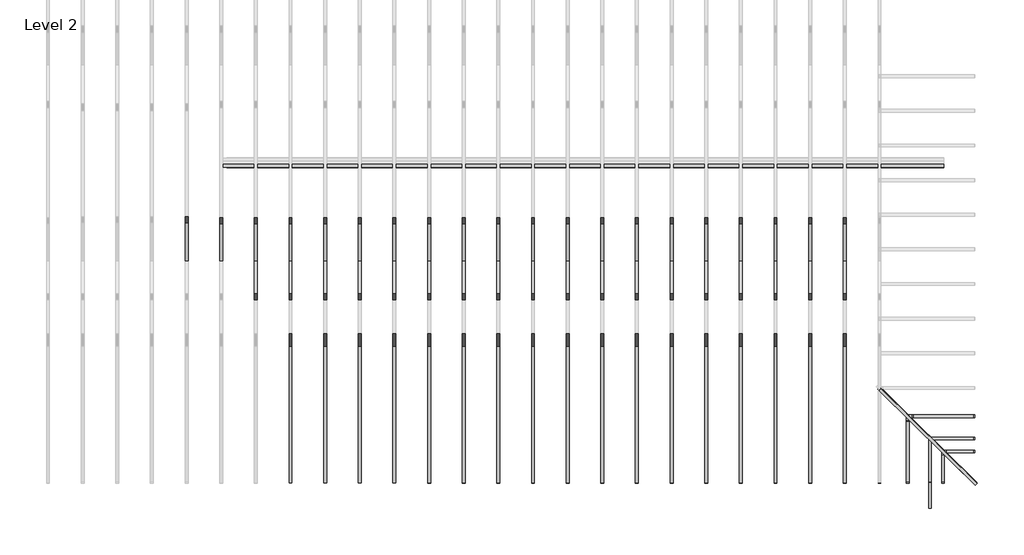
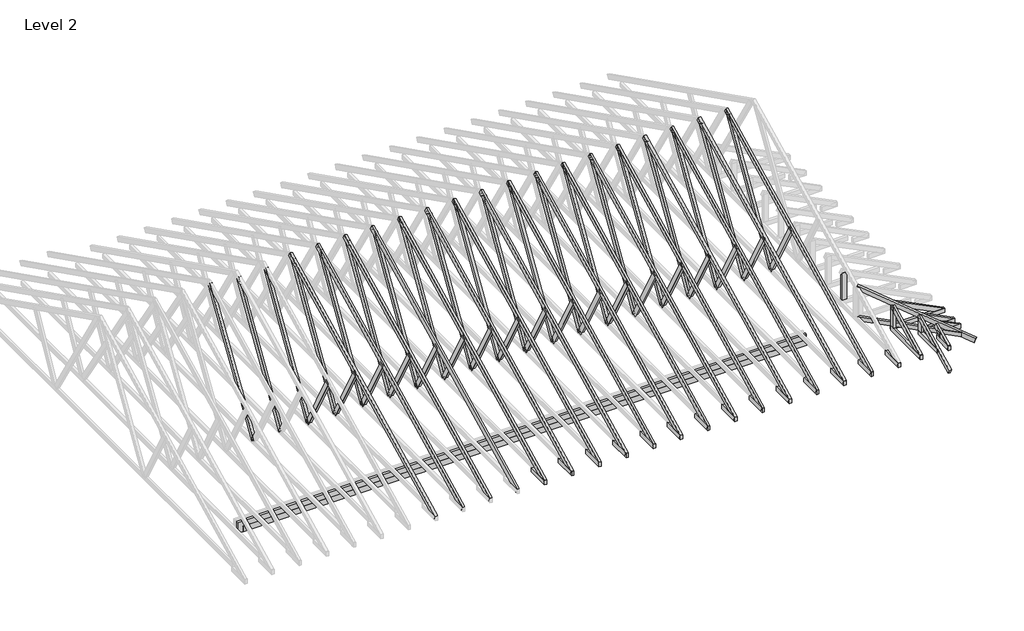
# One storey, part 2 of 5: 92 beams.
"""IFC4 building model written with IfcOpenShell, lengths in millimetres."""

import ifcopenshell
import ifcopenshell.guid

model = None  # the IFC model being written
_history = None  # IfcOwnerHistory: only IFC2X3 demands one
_inside = {}  # id of a spatial element -> (the spatial element, [elements in it])
_under = {}  # id of a project, library or spatial element -> (it, [spatial elements below it])
_declared = {}  # id of a project -> (the project, [libraries it declares])
_typed = {}  # id of a type object -> (the type object, [elements of that type])
_made_of = {}  # id of a material, layer set ... -> (it, [elements and type objects made of it])


def new_model(schema):
    """Start an empty IFC model of exactly this schema.

    Asked for "IFC4X3", IfcOpenShell would pick the latest addendum, in which some entities
    have other attributes; the version numbers below select the first issue.
    IFC2X3 requires an IfcOwnerHistory on every rooted entity: one is made here for all.
    """
    global model, _history
    if schema == "IFC4X3":
        model = ifcopenshell.file(schema_version=(4, 3, 0, 0))
    else:
        model = ifcopenshell.file(schema=schema)
    _inside.clear()
    _under.clear()
    _declared.clear()
    _typed.clear()
    _made_of.clear()
    _history = None
    if model.schema == "IFC2X3":
        org = make("IfcOrganization", Name="unknown")
        user = make(
            "IfcPersonAndOrganization",
            ThePerson=make("IfcPerson", FamilyName="unknown"),
            TheOrganization=org,
        )
        app = make(
            "IfcApplication",
            ApplicationDeveloper=org,
            Version="unknown",
            ApplicationFullName="unknown",
            ApplicationIdentifier="unknown",
        )
        _history = make(
            "IfcOwnerHistory",
            OwningUser=user,
            OwningApplication=app,
            ChangeAction="ADDED",
            CreationDate=0,
        )
    return model


def make(cls, **values):
    """One entity of the class cls with the attributes given. An attribute that is None is left unset."""
    return model.create_entity(
        cls, **{name: value for name, value in values.items() if value is not None}
    )


def rooted(cls, **values):
    """An entity with a GlobalId (a new one), such as an element, a storey or a relation."""
    return make(cls, GlobalId=ifcopenshell.guid.new(), OwnerHistory=_history, **values)


def si_unit(unit_type, name, prefix=None):
    """IfcSIUnit, for example si_unit("LENGTHUNIT", "METRE", prefix="MILLI")."""
    return make("IfcSIUnit", UnitType=unit_type, Prefix=prefix, Name=name)


def assignment(units):
    """IfcUnitAssignment: the units of a project."""
    return None if units is None else make("IfcUnitAssignment", Units=units)


def point(xyz):
    """IfcCartesianPoint."""
    return None if xyz is None else make("IfcCartesianPoint", Coordinates=xyz)


def direction(xyz):
    """IfcDirection."""
    return None if xyz is None else make("IfcDirection", DirectionRatios=xyz)


def frame(location, z_axis=None, x_axis=None):
    """IfcAxis2Placement3D, a coordinate frame: its origin and axes. An axis left out is left unset."""
    return make(
        "IfcAxis2Placement3D",
        Location=point(location),
        Axis=direction(z_axis),
        RefDirection=direction(x_axis),
    )


def origin():
    """The frame at (0, 0, 0) with its axes left unset."""
    return frame((0.0, 0.0, 0.0))


def place(relative_to, where):
    """IfcLocalPlacement: puts the frame where relative to a parent placement (None: the world)."""
    return make(
        "IfcLocalPlacement", PlacementRelTo=relative_to, RelativePlacement=where
    )


def context(
    kind, dimensions, precision=None, world=None, true_north=None, identifier=None
):
    """IfcGeometricRepresentationContext, for example the 3D "Model" context."""
    return make(
        "IfcGeometricRepresentationContext",
        ContextIdentifier=identifier,
        ContextType=kind,
        CoordinateSpaceDimension=dimensions,
        Precision=precision,
        WorldCoordinateSystem=world,
        TrueNorth=true_north,
    )


def project(units=None, contexts=None):
    """IfcProject with its units and contexts."""
    return rooted(
        "IfcProject",
        Name="project",
        RepresentationContexts=contexts,
        UnitsInContext=assignment(units),
    )


def spatial(cls, under=None, at=None, **own):
    """A site, building, storey or space (cls), placed at a placement, below another one or the project."""
    s = rooted(cls, ObjectPlacement=at, **own)
    if under is not None:
        _under.setdefault(under.id(), (under, []))[1].append(s)
    return s


def polyline(points):
    """IfcPolyline through the points."""
    return make("IfcPolyline", Points=[point(p) for p in points])


def outline(outer, holes=None, kind="AREA"):
    """IfcArbitraryClosedProfileDef: a profile drawn as a closed curve; with holes, ...WithVoids."""
    if holes is None:
        return make("IfcArbitraryClosedProfileDef", ProfileType=kind, OuterCurve=outer)
    return make(
        "IfcArbitraryProfileDefWithVoids",
        ProfileType=kind,
        OuterCurve=outer,
        InnerCurves=holes,
    )


def extrude(swept, where, along, depth):
    """IfcExtrudedAreaSolid: the profile swept, set in the frame where, extruded along a direction by depth."""
    return make(
        "IfcExtrudedAreaSolid",
        SweptArea=swept,
        Position=where,
        ExtrudedDirection=direction(along),
        Depth=depth,
    )


def shape(context_of_items, identifier, shape_type, items):
    """IfcShapeRepresentation: the items that make up one representation, for example the "Body"."""
    return make(
        "IfcShapeRepresentation",
        ContextOfItems=context_of_items,
        RepresentationIdentifier=identifier,
        RepresentationType=shape_type,
        Items=items,
    )


def source(mapping_origin, context_of_items, identifier, shape_type, items):
    """IfcRepresentationMap: a shape defined once, which mapped items show again and again."""
    return make(
        "IfcRepresentationMap",
        MappingOrigin=mapping_origin,
        MappedRepresentation=shape(context_of_items, identifier, shape_type, items),
    )


def transform(
    local_origin,
    x_axis=None,
    y_axis=None,
    z_axis=None,
    scale=None,
    scale2=None,
    scale3=None,
    uniform=True,
):
    """IfcCartesianTransformationOperator3D, or its non-uniform kind. x_axis, y_axis, z_axis: its Axis1, 2, 3."""
    if uniform:
        return make(
            "IfcCartesianTransformationOperator3D",
            Axis1=direction(x_axis),
            Axis2=direction(y_axis),
            LocalOrigin=point(local_origin),
            Scale=scale,
            Axis3=direction(z_axis),
        )
    return make(
        "IfcCartesianTransformationOperator3DnonUniform",
        Axis1=direction(x_axis),
        Axis2=direction(y_axis),
        LocalOrigin=point(local_origin),
        Scale=scale,
        Axis3=direction(z_axis),
        Scale2=scale2,
        Scale3=scale3,
    )


def mapped(mapping_source, mapping_target):
    """IfcMappedItem: shows the shape of a source again, moved by a transform."""
    return make(
        "IfcMappedItem", MappingSource=mapping_source, MappingTarget=mapping_target
    )


def made_of(thing, what):
    """Note that an element or type object is made of a material, layer set ...; save() writes the relation."""
    if what is not None:
        _made_of.setdefault(what.id(), (what, []))[1].append(thing)
    return thing


def element(
    cls,
    number,
    at=None,
    inside=None,
    cuts=None,
    type_object=None,
    material=None,
    context=None,
    identifier="Body",
    shape_type=None,
    held_by="IfcProductDefinitionShape",
    body=None,
    shapes=None,
    **own,
):
    """One element of the class cls, such as IfcWall. Its Tag is "e" and its number.

    at: its placement. inside: the storey or other place that contains it. cuts: it is an
    opening in that element (IfcRelVoidsElement). A single representation is given by context,
    identifier, shape_type and body (its items); several are given by shapes. held_by: the class
    of the entity that holds the representations. save() writes the other relations.
    """
    e = rooted(cls, Tag="e%d" % number, ObjectPlacement=at, **own)
    if body is not None:
        shapes = [shape(context, identifier, shape_type, body)]
    if shapes is not None:
        e.Representation = make(held_by, Representations=shapes)
    if inside is not None:
        _inside.setdefault(inside.id(), (inside, []))[1].append(e)
    if cuts is not None:
        rooted(
            "IfcRelVoidsElement", RelatingBuildingElement=cuts, RelatedOpeningElement=e
        )
    if type_object is not None:
        _typed.setdefault(type_object.id(), (type_object, []))[1].append(e)
    return made_of(e, material)


def aggregate(whole, parts):
    """IfcRelAggregates: a whole, such as a stair, and the parts it consists of."""
    return rooted("IfcRelAggregates", RelatingObject=whole, RelatedObjects=parts)


def save(model, path):
    """Write the relations noted so far, then the file.

    IfcRelAggregates (storeys below a building ...), IfcRelContainedInSpatialStructure (elements
    in a storey), IfcRelDefinesByType, IfcRelAssociatesMaterial and IfcRelDeclares: one each for
    every whole, place, type object, material and project.
    """
    for whole, parts in _under.values():
        aggregate(whole, parts)
    for where, things in _inside.values():
        rooted(
            "IfcRelContainedInSpatialStructure",
            RelatedElements=things,
            RelatingStructure=where,
        )
    for kind, things in _typed.values():
        rooted("IfcRelDefinesByType", RelatedObjects=things, RelatingType=kind)
    for what, things in _made_of.values():
        rooted("IfcRelAssociatesMaterial", RelatedObjects=things, RelatingMaterial=what)
    for by, libraries in _declared.values():
        rooted("IfcRelDeclares", RelatingContext=by, RelatedDefinitions=libraries)
    model.write(path)


def beam_7745fe0f(model_context):
    return source(origin(), model_context, "Body", "SweptSolid", [
        extrude(outline(polyline([(393.7, 25.4), (393.7, -25.4), (-393.7, -25.4), (-393.7, 25.4), (393.7, 25.4)])), frame((0.0, 0.0, -50.8), z_axis=(0.0, 0.0, 1.0), x_axis=(1.0, 0.0, 0.0)), (0.0, 0.0, 1.0), 101.6),
    ])


def beam_16181373(model_context):
    return source(origin(), model_context, "Body", "SweptSolid", [
        extrude(outline(polyline([(819.5010489, 25.4), (819.5010489, -25.4), (-821.193698, -25.4), (-821.193698, 25.4), (819.5010489, 25.4)])), frame((0.0, 0.0, -50.8), z_axis=(0.0, 0.0, 1.0), x_axis=(1.0, 0.0, 0.0)), (0.0, 0.0, 1.0), 101.6),
    ])


def beam_e838d316(model_context):
    return source(origin(), model_context, "Body", "SweptSolid", [
        extrude(outline(polyline([(1561.1045551, 25.4), (1561.1045551, -25.4), (-1572.5300502, -25.4), (-1572.5300502, 25.4), (1561.1045551, 25.4)])), frame((0.0, 0.0, -50.8), z_axis=(0.0, 0.0, 1.0), x_axis=(1.0, 0.0, 0.0)), (0.0, 0.0, 1.0), 101.6),
    ])


def beam_6a2c9f8f(model_context):
    return source(origin(), model_context, "Body", "SweptSolid", [
        extrude(outline(polyline([(1599.9543138, 25.4), (1599.9543138, -25.4), (-1584.2465686, -25.4), (-1584.2465686, 25.4), (1599.9543138, 25.4)])), frame((0.0, 0.0, -50.8), z_axis=(0.0, 0.0, 1.0), x_axis=(1.0, 0.0, 0.0)), (0.0, 0.0, 1.0), 101.6),
    ])


def beam_87710fdd(model_context):
    return source(origin(), model_context, "Body", "SweptSolid", [
        extrude(outline(polyline([(147.1272806, 25.4), (147.1272806, -25.4), (-142.875, -25.4), (-142.875, 25.4), (147.1272806, 25.4)])), frame((0.0, 0.0, -50.8), z_axis=(0.0, 0.0, 1.0), x_axis=(1.0, 0.0, 0.0)), (0.0, 0.0, 1.0), 101.6),
    ])


def beam_af5d22dc(model_context):
    return source(origin(), model_context, "Body", "SweptSolid", [
        extrude(outline(polyline([(571.5, 25.4), (571.5, -25.4), (-609.6, -25.4), (-609.6, 25.4), (571.5, 25.4)])), frame((0.0, 0.0, -50.8), z_axis=(0.0, 0.0, 1.0), x_axis=(1.0, 0.0, 0.0)), (0.0, 0.0, 1.0), 101.6),
    ])


def beam_7b8fa6d1(model_context):
    return source(origin(), model_context, "Body", "SweptSolid", [
        extrude(outline(polyline([(270.7395597, 25.4), (270.7395597, -25.4), (-219.9395597, -25.4), (-219.9395597, 25.4), (270.7395597, 25.4)])), frame((0.0, 0.0, -50.8), z_axis=(0.0, 0.0, 1.0), x_axis=(1.0, 0.0, 0.0)), (0.0, 0.0, 1.0), 101.6),
    ])


def beam_42a29ae5(model_context):
    return source(origin(), model_context, "Body", "SweptSolid", [
        extrude(outline(polyline([(270.7395597, -25.4), (-219.9395597, -25.4), (-219.9395597, 25.4), (270.7395597, 25.4), (270.7395597, -25.4)])), frame((0.0, 0.0, -50.8), z_axis=(0.0, 0.0, 1.0), x_axis=(1.0, 0.0, 0.0)), (0.0, 0.0, 1.0), 101.6),
    ])


def beam_11c5b8ca(model_context):
    return source(origin(), model_context, "Body", "SweptSolid", [
        extrude(outline(polyline([(147.1272806, -25.4), (-142.875, -25.4), (-142.875, 25.4), (147.1272806, 25.4), (147.1272806, -25.4)])), frame((0.0, 0.0, -50.8), z_axis=(0.0, 0.0, 1.0), x_axis=(1.0, 0.0, 0.0)), (0.0, 0.0, 1.0), 101.6),
    ])


def beam_5ac0b85f(model_context):
    return source(origin(), model_context, "Body", "SweptSolid", [
        extrude(outline(polyline([(571.5, -25.4), (-584.2, -25.4), (-584.2, 25.4), (571.5, 25.4), (571.5, -25.4)])), frame((0.0, 0.0, -50.8), z_axis=(0.0, 0.0, 1.0), x_axis=(1.0, 0.0, 0.0)), (0.0, 0.0, 1.0), 101.6),
    ])


def beam_99e5442a(model_context):
    return source(origin(), model_context, "Body", "SweptSolid", [
        extrude(outline(polyline([(350.5042173, -25.4), (-295.4519367, -25.4), (-295.4519367, 25.4), (350.5042173, 25.4), (350.5042173, -25.4)])), frame((0.0, 0.0, -50.8), z_axis=(0.0, 0.0, 1.0), x_axis=(1.0, 0.0, 0.0)), (0.0, 0.0, 1.0), 101.6),
    ])


def beam_ec111315(model_context):
    return source(origin(), model_context, "Body", "SweptSolid", [
        extrude(outline(polyline([(279.4, -25.4), (-228.6, -25.4), (-228.6, 25.4), (279.4, 25.4), (279.4, -25.4)])), frame((0.0, 0.0, -50.8), z_axis=(0.0, 0.0, 1.0), x_axis=(1.0, 0.0, 0.0)), (0.0, 0.0, 1.0), 101.6),
    ])


def beam_878446a4(model_context):
    return source(origin(), model_context, "Body", "SweptSolid", [
        extrude(outline(polyline([(63.8057136, 25.4), (63.8057136, -25.4), (-59.553433, -25.4), (-59.553433, 25.4), (63.8057136, 25.4)])), frame((0.0, 0.0, -50.8), z_axis=(0.0, 0.0, 1.0), x_axis=(1.0, 0.0, 0.0)), (0.0, 0.0, 1.0), 101.6),
    ])


def beam_bc99fd75(model_context):
    return source(origin(), model_context, "Body", "SweptSolid", [
        extrude(outline(polyline([(222.3387319, 25.4), (222.3387319, -25.4), (-231.775, -25.4), (-231.775, 25.4), (222.3387319, 25.4)])), frame((0.0, 0.0, -50.8), z_axis=(0.0, 0.0, 1.0), x_axis=(1.0, 0.0, 0.0)), (0.0, 0.0, 1.0), 101.6),
    ])


def beam_efe25585(model_context):
    return source(origin(), model_context, "Body", "SweptSolid", [
        extrude(outline(polyline([(222.3387319, -25.4), (-231.775, -25.4), (-231.775, 25.4), (222.3387319, 25.4), (222.3387319, -25.4)])), frame((0.0, 0.0, -50.8), z_axis=(0.0, 0.0, 1.0), x_axis=(1.0, 0.0, 0.0)), (0.0, 0.0, 1.0), 101.6),
    ])


def beam_dfed05dc(model_context):
    return source(origin(), model_context, "Body", "SweptSolid", [
        extrude(outline(polyline([(63.8057136, -25.4), (-59.553433, -25.4), (-59.553433, 25.4), (63.8057136, 25.4), (63.8057136, -25.4)])), frame((0.0, 0.0, -50.8), z_axis=(0.0, 0.0, 1.0), x_axis=(1.0, 0.0, 0.0)), (0.0, 0.0, 1.0), 101.6),
    ])


def beam_b8261971(model_context):
    return source(origin(), model_context, "Body", "SweptSolid", [
        extrude(outline(polyline([(233.4866591, 25.4), (233.4866591, -25.4), (-1841.8619641, -25.4), (-1841.8619641, 25.4), (233.4866591, 25.4)])), frame((0.0, 0.0, -50.8), z_axis=(0.0, 0.0, 1.0), x_axis=(1.0, 0.0, 0.0)), (0.0, 0.0, 1.0), 101.6),
    ])


def beam_925b2549(model_context):
    return source(origin(), model_context, "Body", "SweptSolid", [
        extrude(outline(polyline([(371.7582386, -25.4), (-368.3, -25.4), (-368.3, 25.4), (371.7582386, 25.4), (371.7582386, -25.4)])), frame((0.0, 0.0, -50.8), z_axis=(0.0, 0.0, 1.0), x_axis=(1.0, 0.0, 0.0)), (0.0, 0.0, 1.0), 101.6),
    ])


def beam_bcf194da(model_context):
    return source(origin(), model_context, "Body", "SweptSolid", [
        extrude(outline(polyline([(6302.375, 25.4), (6302.375, -25.4), (-6429.375, -25.4), (-6429.375, 25.4), (6302.375, 25.4)])), frame((0.0, 0.0, -127.0), z_axis=(0.0, 0.0, 1.0), x_axis=(1.0, 0.0, 0.0)), (0.0, 0.0, 1.0), 254.0),
    ])


def beam_af2566d3(model_context):
    return source(origin(), model_context, "Body", "SweptSolid", [
        extrude(outline(polyline([(6458.3020508, 5.55625), (6458.3020508, -5.55625), (-6159.1479492, -5.55625), (-6159.1479492, 5.55625), (6458.3020508, 5.55625)])), frame((0.0, 0.0, -63.5), z_axis=(0.0, 0.0, 1.0), x_axis=(1.0, 0.0, 0.0)), (0.0, 0.0, 1.0), 127.0),
    ])


model = new_model("IFC4")

# Units and contexts
model_context = context("Model", 3, world=origin())
ifc_project = project(units=[si_unit("LENGTHUNIT", "METRE", prefix="MILLI")], contexts=[model_context])

# Site, building, storey
site = spatial("IfcSite", under=ifc_project)
building = spatial("IfcBuilding", under=site)
storey = spatial("IfcBuildingStorey", under=building, Name="Level 2", Elevation=2768.6)

# Beams
placement = place(None, origin())
element("IfcBeam", 1, ObjectType="Dimension Lumber : BLDG 6241 2X4\" TRUSS MEMBER", at=placement, inside=storey, context=model_context, shape_type="SweptSolid", body=[
    extrude(outline(polyline([(0.0, -50.8), (0.0, 0.0), (6302.3539791, 0.0), (6302.3539791, -50.8), (0.0, -50.8)])), frame((-9901.814829, -5565.5155384, 2678.5857718), z_axis=(0.0, -0.447213595499958, 0.894427190999916), x_axis=(0.0, 0.894427190999916, 0.447213595499958)), (0.0, 0.0, 1.0), 101.6),
])
element("IfcBeam", 2, ObjectType="Dimension Lumber : BLDG 6241 2X4\" TRUSS MEMBER", at=placement, inside=storey, context=model_context, shape_type="SweptSolid", body=[
    extrude(outline(polyline([(0.0, -50.8), (0.0, 0.0), (6302.3539791, 0.0), (6302.3539791, -50.8), (0.0, -50.8)])), frame((-9292.214829, -5565.5155384, 2678.5857718), z_axis=(0.0, -0.447213595499958, 0.894427190999916), x_axis=(0.0, 0.894427190999916, 0.447213595499958)), (0.0, 0.0, 1.0), 101.6),
])
element("IfcBeam", 3, ObjectType="Dimension Lumber : BLDG 6241 2X4\" TRUSS MEMBER", at=placement, inside=storey, context=model_context, shape_type="SweptSolid", body=[
    extrude(outline(polyline([(0.0, -50.8), (0.0, 0.0), (6302.3539791, 0.0), (6302.3539791, -50.8), (0.0, -50.8)])), frame((-8682.614829, -5565.5155384, 2678.5857718), z_axis=(0.0, -0.447213595499958, 0.894427190999916), x_axis=(0.0, 0.894427190999916, 0.447213595499958)), (0.0, 0.0, 1.0), 101.6),
])
element("IfcBeam", 4, ObjectType="Dimension Lumber : BLDG 6241 2X4\" TRUSS MEMBER", at=placement, inside=storey, context=model_context, shape_type="SweptSolid", body=[
    extrude(outline(polyline([(0.0, -50.8), (0.0, 0.0), (6302.3539791, 0.0), (6302.3539791, -50.8), (0.0, -50.8)])), frame((-8073.014829, -5565.5155384, 2678.5857718), z_axis=(0.0, -0.447213595499958, 0.894427190999916), x_axis=(0.0, 0.894427190999916, 0.447213595499958)), (0.0, 0.0, 1.0), 101.6),
])
element("IfcBeam", 5, ObjectType="Dimension Lumber : BLDG 6241 2X4\" TRUSS MEMBER", at=placement, inside=storey, context=model_context, shape_type="SweptSolid", body=[
    extrude(outline(polyline([(0.0, -50.8), (0.0, 0.0), (6302.3539791, 0.0), (6302.3539791, -50.8), (0.0, -50.8)])), frame((-7463.414829, -5565.5155384, 2678.5857718), z_axis=(0.0, -0.447213595499958, 0.8944271909999159), x_axis=(0.0, 0.8944271909999159, 0.447213595499958)), (0.0, 0.0, 1.0), 101.6),
])
element("IfcBeam", 6, ObjectType="Dimension Lumber : BLDG 6241 2X4\" TRUSS MEMBER", at=placement, inside=storey, context=model_context, shape_type="SweptSolid", body=[
    extrude(outline(polyline([(0.0, -50.8), (0.0, 0.0), (6302.3539791, 0.0), (6302.3539791, -50.8), (0.0, -50.8)])), frame((-6853.814829, -5565.5155384, 2678.5857718), z_axis=(0.0, -0.44721359549995776, 0.894427190999916), x_axis=(0.0, 0.894427190999916, 0.44721359549995776)), (0.0, 0.0, 1.0), 101.6),
])
element("IfcBeam", 7, ObjectType="Dimension Lumber : BLDG 6241 2X4\" TRUSS MEMBER", at=placement, inside=storey, context=model_context, shape_type="SweptSolid", body=[
    extrude(outline(polyline([(0.0, -50.8), (0.0, 0.0), (6302.3539791, 0.0), (6302.3539791, -50.8), (0.0, -50.8)])), frame((-6244.214829, -5565.5155384, 2678.5857718), z_axis=(0.0, -0.447213595499958, 0.894427190999916), x_axis=(0.0, 0.894427190999916, 0.447213595499958)), (0.0, 0.0, 1.0), 101.6),
])
element("IfcBeam", 8, ObjectType="Dimension Lumber : BLDG 6241 2X4\" TRUSS MEMBER", at=placement, inside=storey, context=model_context, shape_type="SweptSolid", body=[
    extrude(outline(polyline([(0.0, -50.8), (0.0, 0.0), (6302.3539791, 0.0), (6302.3539791, -50.8), (0.0, -50.8)])), frame((-5634.614829, -5565.5155384, 2678.5857718), z_axis=(0.0, -0.447213595499958, 0.894427190999916), x_axis=(0.0, 0.894427190999916, 0.447213595499958)), (0.0, 0.0, 1.0), 101.6),
])
element("IfcBeam", 9, ObjectType="Dimension Lumber : BLDG 6241 2X4\" TRUSS MEMBER", at=placement, inside=storey, context=model_context, shape_type="SweptSolid", body=[
    extrude(outline(polyline([(0.0, -50.8), (0.0, 0.0), (6302.3539791, 0.0), (6302.3539791, -50.8), (0.0, -50.8)])), frame((-5025.014829, -5565.5155384, 2678.5857718), z_axis=(0.0, -0.447213595499958, 0.894427190999916), x_axis=(0.0, 0.894427190999916, 0.447213595499958)), (0.0, 0.0, 1.0), 101.6),
])
element("IfcBeam", 10, ObjectType="Dimension Lumber : BLDG 6241 2X4\" TRUSS MEMBER", at=placement, inside=storey, context=model_context, shape_type="SweptSolid", body=[
    extrude(outline(polyline([(0.0, -50.8), (0.0, 0.0), (6302.3539791, 0.0), (6302.3539791, -50.8), (0.0, -50.8)])), frame((-4415.414829, -5565.5155384, 2678.5857718), z_axis=(0.0, -0.447213595499958, 0.894427190999916), x_axis=(0.0, 0.894427190999916, 0.447213595499958)), (0.0, 0.0, 1.0), 101.6),
])
element("IfcBeam", 11, ObjectType="Dimension Lumber : BLDG 6241 2X4\" TRUSS MEMBER", at=placement, inside=storey, context=model_context, shape_type="SweptSolid", body=[
    extrude(outline(polyline([(0.0, -50.8), (0.0, 0.0), (6302.3539791, 0.0), (6302.3539791, -50.8), (0.0, -50.8)])), frame((-3805.814829, -5565.5155384, 2678.5857718), z_axis=(0.0, -0.447213595499958, 0.894427190999916), x_axis=(0.0, 0.894427190999916, 0.447213595499958)), (0.0, 0.0, 1.0), 101.6),
])
element("IfcBeam", 12, ObjectType="Dimension Lumber : BLDG 6241 2X4\" TRUSS MEMBER", at=placement, inside=storey, context=model_context, shape_type="SweptSolid", body=[
    extrude(outline(polyline([(0.0, -50.8), (0.0, 0.0), (6302.3539791, 0.0), (6302.3539791, -50.8), (0.0, -50.8)])), frame((-3196.214829, -5565.5155384, 2678.5857718), z_axis=(0.0, -0.447213595499958, 0.894427190999916), x_axis=(0.0, 0.894427190999916, 0.447213595499958)), (0.0, 0.0, 1.0), 101.6),
])
element("IfcBeam", 13, ObjectType="Dimension Lumber : BLDG 6241 2X4\" TRUSS MEMBER", at=placement, inside=storey, context=model_context, shape_type="SweptSolid", body=[
    extrude(outline(polyline([(0.0, -50.8), (0.0, 0.0), (6302.3539791, 0.0), (6302.3539791, -50.8), (0.0, -50.8)])), frame((-2586.614829, -5565.5155384, 2678.5857718), z_axis=(0.0, -0.447213595499958, 0.894427190999916), x_axis=(0.0, 0.894427190999916, 0.447213595499958)), (0.0, 0.0, 1.0), 101.6),
])
element("IfcBeam", 14, ObjectType="Dimension Lumber : BLDG 6241 2X4\" TRUSS MEMBER", at=placement, inside=storey, context=model_context, shape_type="SweptSolid", body=[
    extrude(outline(polyline([(0.0, -50.8), (0.0, 0.0), (6302.3539791, 0.0), (6302.3539791, -50.8), (0.0, -50.8)])), frame((-1977.014829, -5565.5155384, 2678.5857718), z_axis=(0.0, -0.447213595499958, 0.894427190999916), x_axis=(0.0, 0.894427190999916, 0.447213595499958)), (0.0, 0.0, 1.0), 101.6),
])
element("IfcBeam", 15, ObjectType="Dimension Lumber : BLDG 6241 2X4\" TRUSS MEMBER", at=placement, inside=storey, context=model_context, shape_type="SweptSolid", body=[
    extrude(outline(polyline([(0.0, -50.8), (0.0, 0.0), (6302.3539791, 0.0), (6302.3539791, -50.8), (0.0, -50.8)])), frame((-1367.414829, -5565.5155384, 2678.5857718), z_axis=(0.0, -0.447213595499958, 0.894427190999916), x_axis=(0.0, 0.894427190999916, 0.447213595499958)), (0.0, 0.0, 1.0), 101.6),
])
element("IfcBeam", 16, ObjectType="Dimension Lumber : BLDG 6241 2X4\" TRUSS MEMBER", at=placement, inside=storey, context=model_context, shape_type="SweptSolid", body=[
    extrude(outline(polyline([(0.0, -50.8), (0.0, 0.0), (6302.3539791, 0.0), (6302.3539791, -50.8), (0.0, -50.8)])), frame((-757.814829, -5565.5155384, 2678.5857718), z_axis=(0.0, -0.447213595499958, 0.8944271909999159), x_axis=(0.0, 0.8944271909999159, 0.447213595499958)), (0.0, 0.0, 1.0), 101.6),
])
element("IfcBeam", 17, ObjectType="Dimension Lumber : BLDG 6241 2X4\" TRUSS MEMBER", at=placement, inside=storey, context=model_context, shape_type="SweptSolid", body=[
    extrude(outline(polyline([(0.0, -50.8), (0.0, 0.0), (6302.3539791, 0.0), (6302.3539791, -50.8), (0.0, -50.8)])), frame((-148.214829, -5565.5155384, 2678.5857718), z_axis=(0.0, -0.44721359549995776, 0.894427190999916), x_axis=(0.0, 0.894427190999916, 0.44721359549995776)), (0.0, 0.0, 1.0), 101.6),
])
element("IfcBeam", 18, ObjectType="Dimension Lumber : BLDG 6241 2X4\" TRUSS MEMBER", at=placement, inside=storey, context=model_context, shape_type="SweptSolid", body=[
    extrude(outline(polyline([(0.0, -50.8000001), (0.0, 0.0), (2518.7475141, -1e-07), (2518.747514, -50.8), (0.0, -50.8000001)])), frame((497.0810747, -3923.9012552, 3516.9362486), z_axis=(0.22183093198504453, -0.25320527715849106, 0.9416358772018718), x_axis=(0.6716162760239294, -0.6604274920267077, -0.3358081380119639)), (0.0, 0.0, 1.0), 101.6),
])
element("IfcBeam", 19, ObjectType="Dimension Lumber : BLDG 6241 2X4\" TRUSS MEMBER", at=placement, inside=storey, context=model_context, shape_type="SweptSolid", body=[
    extrude(outline(polyline([(0.0, -50.8), (0.0, 0.0), (1203.6219076, 0.0), (1203.6219076, -50.8), (0.0, -50.8)])), frame((2112.5153243, -4456.9715886, 2680.3426701), z_axis=(0.44721359549995937, 0.0, 0.8944271909999152), x_axis=(-0.8944271909999152, 0.0, 0.44721359549995937)), (0.0, 0.0, 1.0), 101.6),
])
element("IfcBeam", 20, ObjectType="Dimension Lumber : BLDG 6241 2X4\" TRUSS MEMBER", at=placement, inside=storey, context=model_context, shape_type="SweptSolid", body=[
    extrude(outline(polyline([(0.0, -50.8), (0.0, 0.0), (844.55, 0.0), (844.55, -50.8), (0.0, -50.8)])), frame((2117.2589031, -4850.6715886, 2677.9708807), z_axis=(0.4472135954999599, 0.0, 0.894427190999915), x_axis=(-0.894427190999915, 0.0, 0.4472135954999599)), (0.0, 0.0, 1.0), 101.6),
])
element("IfcBeam", 21, ObjectType="Dimension Lumber : BLDG 6241 2X4\" TRUSS MEMBER", at=placement, inside=storey, context=model_context, shape_type="SweptSolid", body=[
    extrude(outline(polyline([(0.0, 50.8), (1203.6219076, 50.8), (1203.6219076, 0.0), (0.0, 0.0), (0.0, 50.8)])), frame((1007.485171, -5562.001742, 2680.3426701), z_axis=(0.0, -0.44721359549995937, 0.8944271909999152), x_axis=(0.0, 0.8944271909999152, 0.44721359549995937)), (0.0, 0.0, 1.0), 101.6),
])
element("IfcBeam", 22, ObjectType="Dimension Lumber : BLDG 6241 2X4\" TRUSS MEMBER", at=placement, inside=storey, context=model_context, shape_type="SweptSolid", body=[
    extrude(outline(polyline([(0.0, 50.8), (1334.5727744, 50.8), (1334.5727744, 0.0), (0.0, 0.0), (0.0, 50.8)])), frame((1401.185171, -6005.0350144, 2458.8260339), z_axis=(0.0, -0.4472135954999599, 0.894427190999915), x_axis=(0.0, 0.894427190999915, 0.4472135954999599)), (0.0, 0.0, 1.0), 101.6),
])
element("IfcBeam", 23, ObjectType="Dimension Lumber : BLDG 6241 2X4\" TRUSS MEMBER", at=placement, inside=storey, context=model_context, shape_type="SweptSolid", body=[
    extrude(outline(polyline([(0.0, -50.8), (0.0, 0.0), (546.1, 0.0), (546.1, -50.8), (0.0, -50.8)])), frame((2116.9461224, -5079.2715886, 2678.127271), z_axis=(0.4472135954999593, 0.0, 0.8944271909999153), x_axis=(-0.8944271909999153, 0.0, 0.4472135954999593)), (0.0, 0.0, 1.0), 101.6),
])
element("IfcBeam", 24, ObjectType="Dimension Lumber : BLDG 6241 2X4\" TRUSS MEMBER", at=placement, inside=storey, context=model_context, shape_type="SweptSolid", body=[
    extrude(outline(polyline([(0.0, 50.8), (546.1, 50.8), (546.1, 0.0), (0.0, 0.0), (0.0, 50.8)])), frame((1629.785171, -5566.43254, 2678.127271), z_axis=(0.0, -0.4472135954999592, 0.8944271909999153), x_axis=(0.0, 0.8944271909999153, 0.4472135954999592)), (0.0, 0.0, 1.0), 101.6),
])
beam_shape = beam_7745fe0f(model_context)
element("IfcBeam", 25, ObjectType="Dimension Lumber : BLDG 6241 2X4\" TRUSS MEMBER", at=placement, inside=storey, context=model_context, shape_type="MappedRepresentation", body=[
    mapped(beam_shape, transform((1769.485171, -4825.2715886, 2728.7708807), x_axis=(1.0, 0.0, 0.0), y_axis=(0.0, 1.0, 0.0), z_axis=(0.0, 0.0, 1.0))),
])
beam_2_shape = beam_16181373(model_context)
element("IfcBeam", 26, ObjectType="Dimension Lumber : BLDG 6241 2X4\" TRUSS MEMBER", at=placement, inside=storey, context=model_context, shape_type="MappedRepresentation", body=[
    mapped(beam_2_shape, transform((-10486.014829, -2095.6213634, 3552.5770493), x_axis=(0.0, -0.4803172630852174, 0.8770948220017754), y_axis=(-1.0, 0.0, 0.0), z_axis=(0.0, -0.8770948220017754, -0.4803172630852174))),
])
element("IfcBeam", 27, ObjectType="Dimension Lumber : BLDG 6241 2X4\" TRUSS MEMBER", at=placement, inside=storey, context=model_context, shape_type="MappedRepresentation", body=[
    mapped(beam_2_shape, transform((-9876.414829, -2095.6213634, 3552.5770493), x_axis=(0.0, -0.4803172630852174, 0.8770948220017754), y_axis=(-1.0, 0.0, 0.0), z_axis=(0.0, -0.8770948220017754, -0.4803172630852174))),
])
element("IfcBeam", 28, ObjectType="Dimension Lumber : BLDG 6241 2X4\" TRUSS MEMBER", at=placement, inside=storey, context=model_context, shape_type="MappedRepresentation", body=[
    mapped(beam_2_shape, transform((-9266.814829, -2095.6213634, 3552.5770493), x_axis=(0.0, -0.4803172630852174, 0.8770948220017754), y_axis=(-1.0, 0.0, 0.0), z_axis=(0.0, -0.8770948220017754, -0.4803172630852174))),
])
element("IfcBeam", 29, ObjectType="Dimension Lumber : BLDG 6241 2X4\" TRUSS MEMBER", at=placement, inside=storey, context=model_context, shape_type="MappedRepresentation", body=[
    mapped(beam_2_shape, transform((-8657.214829, -2095.6213634, 3552.5770493), x_axis=(0.0, -0.4803172630852174, 0.8770948220017754), y_axis=(-1.0, 0.0, 0.0), z_axis=(0.0, -0.8770948220017754, -0.4803172630852174))),
])
element("IfcBeam", 30, ObjectType="Dimension Lumber : BLDG 6241 2X4\" TRUSS MEMBER", at=placement, inside=storey, context=model_context, shape_type="MappedRepresentation", body=[
    mapped(beam_2_shape, transform((-8047.614829, -2095.6213634, 3552.5770493), x_axis=(0.0, -0.4803172630852174, 0.8770948220017754), y_axis=(-1.0, 0.0, 0.0), z_axis=(0.0, -0.8770948220017754, -0.4803172630852174))),
])
element("IfcBeam", 31, ObjectType="Dimension Lumber : BLDG 6241 2X4\" TRUSS MEMBER", at=placement, inside=storey, context=model_context, shape_type="MappedRepresentation", body=[
    mapped(beam_2_shape, transform((-7438.014829, -2095.6213634, 3552.5770493), x_axis=(0.0, -0.4803172630852174, 0.8770948220017754), y_axis=(-1.0, 0.0, 0.0), z_axis=(0.0, -0.8770948220017754, -0.4803172630852174))),
])
element("IfcBeam", 32, ObjectType="Dimension Lumber : BLDG 6241 2X4\" TRUSS MEMBER", at=placement, inside=storey, context=model_context, shape_type="MappedRepresentation", body=[
    mapped(beam_2_shape, transform((-6828.414829, -2095.6213634, 3552.5770493), x_axis=(0.0, -0.4803172630852174, 0.8770948220017754), y_axis=(-1.0, 0.0, 0.0), z_axis=(0.0, -0.8770948220017754, -0.4803172630852174))),
])
element("IfcBeam", 33, ObjectType="Dimension Lumber : BLDG 6241 2X4\" TRUSS MEMBER", at=placement, inside=storey, context=model_context, shape_type="MappedRepresentation", body=[
    mapped(beam_2_shape, transform((-6218.814829, -2095.6213634, 3552.5770493), x_axis=(0.0, -0.4803172630852174, 0.8770948220017754), y_axis=(-1.0, 0.0, 0.0), z_axis=(0.0, -0.8770948220017754, -0.4803172630852174))),
])
element("IfcBeam", 34, ObjectType="Dimension Lumber : BLDG 6241 2X4\" TRUSS MEMBER", at=placement, inside=storey, context=model_context, shape_type="MappedRepresentation", body=[
    mapped(beam_2_shape, transform((-5609.214829, -2095.6213634, 3552.5770493), x_axis=(0.0, -0.4803172630852174, 0.8770948220017754), y_axis=(-1.0, 0.0, 0.0), z_axis=(0.0, -0.8770948220017754, -0.4803172630852174))),
])
element("IfcBeam", 35, ObjectType="Dimension Lumber : BLDG 6241 2X4\" TRUSS MEMBER", at=placement, inside=storey, context=model_context, shape_type="MappedRepresentation", body=[
    mapped(beam_2_shape, transform((-4999.614829, -2095.6213634, 3552.5770493), x_axis=(0.0, -0.4803172630852174, 0.8770948220017754), y_axis=(-1.0, 0.0, 0.0), z_axis=(0.0, -0.8770948220017754, -0.4803172630852174))),
])
element("IfcBeam", 36, ObjectType="Dimension Lumber : BLDG 6241 2X4\" TRUSS MEMBER", at=placement, inside=storey, context=model_context, shape_type="MappedRepresentation", body=[
    mapped(beam_2_shape, transform((-4390.014829, -2095.6213634, 3552.5770493), x_axis=(0.0, -0.4803172630852174, 0.8770948220017754), y_axis=(-1.0, 0.0, 0.0), z_axis=(0.0, -0.8770948220017754, -0.4803172630852174))),
])
element("IfcBeam", 37, ObjectType="Dimension Lumber : BLDG 6241 2X4\" TRUSS MEMBER", at=placement, inside=storey, context=model_context, shape_type="MappedRepresentation", body=[
    mapped(beam_2_shape, transform((-3780.414829, -2095.6213634, 3552.5770493), x_axis=(0.0, -0.4803172630852174, 0.8770948220017754), y_axis=(-1.0, 0.0, 0.0), z_axis=(0.0, -0.8770948220017754, -0.4803172630852174))),
])
element("IfcBeam", 38, ObjectType="Dimension Lumber : BLDG 6241 2X4\" TRUSS MEMBER", at=placement, inside=storey, context=model_context, shape_type="MappedRepresentation", body=[
    mapped(beam_2_shape, transform((-3170.814829, -2095.6213634, 3552.5770493), x_axis=(0.0, -0.4803172630852174, 0.8770948220017754), y_axis=(-1.0, 0.0, 0.0), z_axis=(0.0, -0.8770948220017754, -0.4803172630852174))),
])
element("IfcBeam", 39, ObjectType="Dimension Lumber : BLDG 6241 2X4\" TRUSS MEMBER", at=placement, inside=storey, context=model_context, shape_type="MappedRepresentation", body=[
    mapped(beam_2_shape, transform((-2561.214829, -2095.6213634, 3552.5770493), x_axis=(0.0, -0.4803172630852174, 0.8770948220017754), y_axis=(-1.0, 0.0, 0.0), z_axis=(0.0, -0.8770948220017754, -0.4803172630852174))),
])
element("IfcBeam", 40, ObjectType="Dimension Lumber : BLDG 6241 2X4\" TRUSS MEMBER", at=placement, inside=storey, context=model_context, shape_type="MappedRepresentation", body=[
    mapped(beam_2_shape, transform((-1951.614829, -2095.6213634, 3552.5770493), x_axis=(0.0, -0.4803172630852174, 0.8770948220017754), y_axis=(-1.0, 0.0, 0.0), z_axis=(0.0, -0.8770948220017754, -0.4803172630852174))),
])
element("IfcBeam", 41, ObjectType="Dimension Lumber : BLDG 6241 2X4\" TRUSS MEMBER", at=placement, inside=storey, context=model_context, shape_type="MappedRepresentation", body=[
    mapped(beam_2_shape, transform((-1342.014829, -2095.6213634, 3552.5770493), x_axis=(0.0, -0.4803172630852174, 0.8770948220017754), y_axis=(-1.0, 0.0, 0.0), z_axis=(0.0, -0.8770948220017754, -0.4803172630852174))),
])
element("IfcBeam", 42, ObjectType="Dimension Lumber : BLDG 6241 2X4\" TRUSS MEMBER", at=placement, inside=storey, context=model_context, shape_type="MappedRepresentation", body=[
    mapped(beam_2_shape, transform((-732.414829, -2095.6213634, 3552.5770493), x_axis=(0.0, -0.4803172630852174, 0.8770948220017754), y_axis=(-1.0, 0.0, 0.0), z_axis=(0.0, -0.8770948220017754, -0.4803172630852174))),
])
element("IfcBeam", 43, ObjectType="Dimension Lumber : BLDG 6241 2X4\" TRUSS MEMBER", at=placement, inside=storey, context=model_context, shape_type="MappedRepresentation", body=[
    mapped(beam_2_shape, transform((-122.814829, -2095.6213634, 3552.5770493), x_axis=(0.0, -0.4803172630852174, 0.8770948220017754), y_axis=(-1.0, 0.0, 0.0), z_axis=(0.0, -0.8770948220017754, -0.4803172630852174))),
])
beam_3_shape = beam_e838d316(model_context)
element("IfcBeam", 44, ObjectType="Dimension Lumber : BLDG 6241 2X4\" TRUSS MEMBER", at=placement, inside=storey, context=model_context, shape_type="MappedRepresentation", body=[
    mapped(beam_3_shape, transform((-11095.614829, -880.0831247, 4160.3461686), x_axis=(0.0, -0.5257715142502325, -0.8506258371358218), y_axis=(-1.0, 0.0, 0.0), z_axis=(0.0, 0.8506258371358218, -0.5257715142502325))),
])
element("IfcBeam", 45, ObjectType="Dimension Lumber : BLDG 6241 2X4\" TRUSS MEMBER", at=placement, inside=storey, context=model_context, shape_type="MappedRepresentation", body=[
    mapped(beam_3_shape, transform((-10486.014829, -880.0831247, 4160.3461686), x_axis=(0.0, -0.5257715142502325, -0.8506258371358218), y_axis=(-1.0, 0.0, 0.0), z_axis=(0.0, 0.8506258371358218, -0.5257715142502325))),
])
element("IfcBeam", 46, ObjectType="Dimension Lumber : BLDG 6241 2X4\" TRUSS MEMBER", at=placement, inside=storey, context=model_context, shape_type="MappedRepresentation", body=[
    mapped(beam_3_shape, transform((-9876.414829, -880.0831247, 4160.3461686), x_axis=(0.0, -0.5257715142502325, -0.8506258371358218), y_axis=(-1.0, 0.0, 0.0), z_axis=(0.0, 0.8506258371358218, -0.5257715142502325))),
])
element("IfcBeam", 47, ObjectType="Dimension Lumber : BLDG 6241 2X4\" TRUSS MEMBER", at=placement, inside=storey, context=model_context, shape_type="MappedRepresentation", body=[
    mapped(beam_3_shape, transform((-9266.814829, -880.0831247, 4160.3461686), x_axis=(0.0, -0.5257715142502325, -0.8506258371358218), y_axis=(-1.0, 0.0, 0.0), z_axis=(0.0, 0.8506258371358218, -0.5257715142502325))),
])
element("IfcBeam", 48, ObjectType="Dimension Lumber : BLDG 6241 2X4\" TRUSS MEMBER", at=placement, inside=storey, context=model_context, shape_type="MappedRepresentation", body=[
    mapped(beam_3_shape, transform((-8657.214829, -880.0831247, 4160.3461686), x_axis=(0.0, -0.5257715142502325, -0.8506258371358218), y_axis=(-1.0, 0.0, 0.0), z_axis=(0.0, 0.8506258371358218, -0.5257715142502325))),
])
element("IfcBeam", 49, ObjectType="Dimension Lumber : BLDG 6241 2X4\" TRUSS MEMBER", at=placement, inside=storey, context=model_context, shape_type="MappedRepresentation", body=[
    mapped(beam_3_shape, transform((-8047.614829, -880.0831247, 4160.3461686), x_axis=(0.0, -0.5257715142502325, -0.8506258371358218), y_axis=(-1.0, 0.0, 0.0), z_axis=(0.0, 0.8506258371358218, -0.5257715142502325))),
])
element("IfcBeam", 50, ObjectType="Dimension Lumber : BLDG 6241 2X4\" TRUSS MEMBER", at=placement, inside=storey, context=model_context, shape_type="MappedRepresentation", body=[
    mapped(beam_3_shape, transform((-7438.014829, -880.0831247, 4160.3461686), x_axis=(0.0, -0.5257715142502325, -0.8506258371358218), y_axis=(-1.0, 0.0, 0.0), z_axis=(0.0, 0.8506258371358218, -0.5257715142502325))),
])
element("IfcBeam", 51, ObjectType="Dimension Lumber : BLDG 6241 2X4\" TRUSS MEMBER", at=placement, inside=storey, context=model_context, shape_type="MappedRepresentation", body=[
    mapped(beam_3_shape, transform((-6828.414829, -880.0831247, 4160.3461686), x_axis=(0.0, -0.5257715142502325, -0.8506258371358218), y_axis=(-1.0, 0.0, 0.0), z_axis=(0.0, 0.8506258371358218, -0.5257715142502325))),
])
element("IfcBeam", 52, ObjectType="Dimension Lumber : BLDG 6241 2X4\" TRUSS MEMBER", at=placement, inside=storey, context=model_context, shape_type="MappedRepresentation", body=[
    mapped(beam_3_shape, transform((-6218.814829, -880.0831247, 4160.3461686), x_axis=(0.0, -0.5257715142502325, -0.8506258371358218), y_axis=(-1.0, 0.0, 0.0), z_axis=(0.0, 0.8506258371358218, -0.5257715142502325))),
])
element("IfcBeam", 53, ObjectType="Dimension Lumber : BLDG 6241 2X4\" TRUSS MEMBER", at=placement, inside=storey, context=model_context, shape_type="MappedRepresentation", body=[
    mapped(beam_3_shape, transform((-5609.214829, -880.0831247, 4160.3461686), x_axis=(0.0, -0.5257715142502325, -0.8506258371358218), y_axis=(-1.0, 0.0, 0.0), z_axis=(0.0, 0.8506258371358218, -0.5257715142502325))),
])
element("IfcBeam", 54, ObjectType="Dimension Lumber : BLDG 6241 2X4\" TRUSS MEMBER", at=placement, inside=storey, context=model_context, shape_type="MappedRepresentation", body=[
    mapped(beam_3_shape, transform((-4999.614829, -880.0831247, 4160.3461686), x_axis=(0.0, -0.5257715142502325, -0.8506258371358218), y_axis=(-1.0, 0.0, 0.0), z_axis=(0.0, 0.8506258371358218, -0.5257715142502325))),
])
element("IfcBeam", 55, ObjectType="Dimension Lumber : BLDG 6241 2X4\" TRUSS MEMBER", at=placement, inside=storey, context=model_context, shape_type="MappedRepresentation", body=[
    mapped(beam_3_shape, transform((-4390.014829, -880.0831247, 4160.3461686), x_axis=(0.0, -0.5257715142502325, -0.8506258371358218), y_axis=(-1.0, 0.0, 0.0), z_axis=(0.0, 0.8506258371358218, -0.5257715142502325))),
])
element("IfcBeam", 56, ObjectType="Dimension Lumber : BLDG 6241 2X4\" TRUSS MEMBER", at=placement, inside=storey, context=model_context, shape_type="MappedRepresentation", body=[
    mapped(beam_3_shape, transform((-3780.414829, -880.0831247, 4160.3461686), x_axis=(0.0, -0.5257715142502325, -0.8506258371358218), y_axis=(-1.0, 0.0, 0.0), z_axis=(0.0, 0.8506258371358218, -0.5257715142502325))),
])
element("IfcBeam", 57, ObjectType="Dimension Lumber : BLDG 6241 2X4\" TRUSS MEMBER", at=placement, inside=storey, context=model_context, shape_type="MappedRepresentation", body=[
    mapped(beam_3_shape, transform((-3170.814829, -880.0831247, 4160.3461686), x_axis=(0.0, -0.5257715142502325, -0.8506258371358218), y_axis=(-1.0, 0.0, 0.0), z_axis=(0.0, 0.8506258371358218, -0.5257715142502325))),
])
element("IfcBeam", 58, ObjectType="Dimension Lumber : BLDG 6241 2X4\" TRUSS MEMBER", at=placement, inside=storey, context=model_context, shape_type="MappedRepresentation", body=[
    mapped(beam_3_shape, transform((-2561.214829, -880.0831247, 4160.3461686), x_axis=(0.0, -0.5257715142502325, -0.8506258371358218), y_axis=(-1.0, 0.0, 0.0), z_axis=(0.0, 0.8506258371358218, -0.5257715142502325))),
])
element("IfcBeam", 59, ObjectType="Dimension Lumber : BLDG 6241 2X4\" TRUSS MEMBER", at=placement, inside=storey, context=model_context, shape_type="MappedRepresentation", body=[
    mapped(beam_3_shape, transform((-1951.614829, -880.0831247, 4160.3461686), x_axis=(0.0, -0.5257715142502325, -0.8506258371358218), y_axis=(-1.0, 0.0, 0.0), z_axis=(0.0, 0.8506258371358218, -0.5257715142502325))),
])
element("IfcBeam", 60, ObjectType="Dimension Lumber : BLDG 6241 2X4\" TRUSS MEMBER", at=placement, inside=storey, context=model_context, shape_type="MappedRepresentation", body=[
    mapped(beam_3_shape, transform((-1342.014829, -880.0831247, 4160.3461686), x_axis=(0.0, -0.5257715142502325, -0.8506258371358218), y_axis=(-1.0, 0.0, 0.0), z_axis=(0.0, 0.8506258371358218, -0.5257715142502325))),
])
element("IfcBeam", 61, ObjectType="Dimension Lumber : BLDG 6241 2X4\" TRUSS MEMBER", at=placement, inside=storey, context=model_context, shape_type="MappedRepresentation", body=[
    mapped(beam_3_shape, transform((-732.414829, -880.0831247, 4160.3461686), x_axis=(0.0, -0.5257715142502325, -0.8506258371358218), y_axis=(-1.0, 0.0, 0.0), z_axis=(0.0, 0.8506258371358218, -0.5257715142502325))),
])
element("IfcBeam", 62, ObjectType="Dimension Lumber : BLDG 6241 2X4\" TRUSS MEMBER", at=placement, inside=storey, context=model_context, shape_type="MappedRepresentation", body=[
    mapped(beam_3_shape, transform((-122.814829, -880.0831247, 4160.3461686), x_axis=(0.0, -0.5257715142502325, -0.8506258371358218), y_axis=(-1.0, 0.0, 0.0), z_axis=(0.0, 0.8506258371358218, -0.5257715142502325))),
])
beam_4_shape = beam_6a2c9f8f(model_context)
element("IfcBeam", 63, ObjectType="Dimension Lumber : BLDG 6241 2X4\" TRUSS MEMBER", at=placement, inside=storey, context=model_context, shape_type="MappedRepresentation", body=[
    mapped(beam_4_shape, transform((-11705.214829, -844.5384628, 4185.1853738), x_axis=(0.0, -0.5348644598757986, -0.8449378731964677), y_axis=(-1.0, 0.0, 0.0), z_axis=(0.0, 0.8449378731964677, -0.5348644598757986))),
])
beam_5_shape = beam_87710fdd(model_context)
element("IfcBeam", 64, ObjectType="Dimension Lumber : BLDG 6241 2X4\" TRUSS MEMBER", at=placement, inside=storey, context=model_context, shape_type="MappedRepresentation", body=[
    mapped(beam_5_shape, transform((1451.985171, -4825.2715886, 2924.5288734), x_axis=(0.0, 0.0, 1.0), y_axis=(0.0, -1.0, 0.0), z_axis=(1.0, 0.0, 0.0))),
])
beam_6_shape = beam_af5d22dc(model_context)
element("IfcBeam", 65, ObjectType="Dimension Lumber : BLDG 6241 2X4\" TRUSS MEMBER", at=placement, inside=storey, context=model_context, shape_type="MappedRepresentation", body=[
    mapped(beam_6_shape, transform((1591.685171, -4431.5715886, 2728.7708807), x_axis=(1.0, 0.0, 0.0), y_axis=(0.0, 1.0, 0.0), z_axis=(0.0, 0.0, 1.0))),
])
beam_7_shape = beam_7b8fa6d1(model_context)
element("IfcBeam", 66, ObjectType="Dimension Lumber : BLDG 6241 2X4\" TRUSS MEMBER", at=placement, inside=storey, context=model_context, shape_type="MappedRepresentation", body=[
    mapped(beam_7_shape, transform((1058.285171, -4431.5715886, 2999.5104403), x_axis=(0.0, 0.0, 1.0), y_axis=(0.0, -1.0, 0.0), z_axis=(1.0, 0.0, 0.0))),
])
beam_8_shape = beam_42a29ae5(model_context)
element("IfcBeam", 67, ObjectType="Dimension Lumber : BLDG 6241 2X4\" TRUSS MEMBER", at=placement, inside=storey, context=model_context, shape_type="MappedRepresentation", body=[
    mapped(beam_8_shape, transform((982.085171, -4507.7715886, 2999.5104403), x_axis=(0.0, 0.0, 1.0), y_axis=(-1.0, 0.0, 0.0), z_axis=(0.0, -1.0, 0.0))),
])
beam_9_shape = beam_11c5b8ca(model_context)
element("IfcBeam", 68, ObjectType="Dimension Lumber : BLDG 6241 2X4\" TRUSS MEMBER", at=placement, inside=storey, context=model_context, shape_type="MappedRepresentation", body=[
    mapped(beam_9_shape, transform((1375.785171, -4901.4715886, 2924.5288734), x_axis=(0.0, 0.0, 1.0), y_axis=(-1.0, 0.0, 0.0), z_axis=(0.0, -1.0, 0.0))),
])
beam_10_shape = beam_5ac0b85f(model_context)
element("IfcBeam", 69, ObjectType="Dimension Lumber : BLDG 6241 2X4\" TRUSS MEMBER", at=placement, inside=storey, context=model_context, shape_type="MappedRepresentation", body=[
    mapped(beam_10_shape, transform((982.085171, -5041.1715886, 2728.7708807), x_axis=(0.0, -1.0, 0.0), y_axis=(1.0, 0.0, 0.0), z_axis=(0.0, 0.0, 1.0))),
])
beam_11_shape = beam_99e5442a(model_context)
element("IfcBeam", 70, ObjectType="Dimension Lumber : BLDG 6241 2X4\" TRUSS MEMBER", at=placement, inside=storey, context=model_context, shape_type="MappedRepresentation", body=[
    mapped(beam_11_shape, transform((562.985171, -3326.6715886, 3165.6519367), x_axis=(0.0, 0.0, 1.0), y_axis=(0.0, -1.0, 0.0), z_axis=(1.0, 0.0, 0.0))),
])
beam_12_shape = beam_ec111315(model_context)
element("IfcBeam", 71, ObjectType="Dimension Lumber : BLDG 6241 2X4\" TRUSS MEMBER", at=placement, inside=storey, context=model_context, shape_type="MappedRepresentation", body=[
    mapped(beam_12_shape, transform((-7438.014829, -5384.0715886, 2717.8), x_axis=(0.0, 1.0, 0.0), y_axis=(-1.0, 0.0, 0.0), z_axis=(0.0, 0.0, 1.0))),
])
element("IfcBeam", 72, ObjectType="Dimension Lumber : BLDG 6241 2X4\" TRUSS MEMBER", at=placement, inside=storey, context=model_context, shape_type="MappedRepresentation", body=[
    mapped(beam_12_shape, transform((-6828.414829, -5384.0715886, 2717.8), x_axis=(0.0, 1.0, 0.0), y_axis=(-1.0, 0.0, 0.0), z_axis=(0.0, 0.0, 1.0))),
])
element("IfcBeam", 73, ObjectType="Dimension Lumber : BLDG 6241 2X4\" TRUSS MEMBER", at=placement, inside=storey, context=model_context, shape_type="MappedRepresentation", body=[
    mapped(beam_12_shape, transform((-6218.814829, -5384.0715886, 2717.8), x_axis=(0.0, 1.0, 0.0), y_axis=(-1.0, 0.0, 0.0), z_axis=(0.0, 0.0, 1.0))),
])
element("IfcBeam", 74, ObjectType="Dimension Lumber : BLDG 6241 2X4\" TRUSS MEMBER", at=placement, inside=storey, context=model_context, shape_type="MappedRepresentation", body=[
    mapped(beam_12_shape, transform((-5609.214829, -5384.0715886, 2717.8), x_axis=(0.0, 1.0, 0.0), y_axis=(-1.0, 0.0, 0.0), z_axis=(0.0, 0.0, 1.0))),
])
element("IfcBeam", 75, ObjectType="Dimension Lumber : BLDG 6241 2X4\" TRUSS MEMBER", at=placement, inside=storey, context=model_context, shape_type="MappedRepresentation", body=[
    mapped(beam_12_shape, transform((-4999.614829, -5384.0715886, 2717.8), x_axis=(0.0, 1.0, 0.0), y_axis=(-1.0, 0.0, 0.0), z_axis=(0.0, 0.0, 1.0))),
])
element("IfcBeam", 76, ObjectType="Dimension Lumber : BLDG 6241 2X4\" TRUSS MEMBER", at=placement, inside=storey, context=model_context, shape_type="MappedRepresentation", body=[
    mapped(beam_12_shape, transform((-4390.014829, -5384.0715886, 2717.8), x_axis=(0.0, 1.0, 0.0), y_axis=(-1.0, 0.0, 0.0), z_axis=(0.0, 0.0, 1.0))),
])
element("IfcBeam", 77, ObjectType="Dimension Lumber : BLDG 6241 2X4\" TRUSS MEMBER", at=placement, inside=storey, context=model_context, shape_type="MappedRepresentation", body=[
    mapped(beam_12_shape, transform((-3780.414829, -5384.0715886, 2717.8), x_axis=(0.0, 1.0, 0.0), y_axis=(-1.0, 0.0, 0.0), z_axis=(0.0, 0.0, 1.0))),
])
element("IfcBeam", 78, ObjectType="Dimension Lumber : BLDG 6241 2X4\" TRUSS MEMBER", at=placement, inside=storey, context=model_context, shape_type="MappedRepresentation", body=[
    mapped(beam_12_shape, transform((-3170.814829, -5384.0715886, 2717.8), x_axis=(0.0, 1.0, 0.0), y_axis=(-1.0, 0.0, 0.0), z_axis=(0.0, 0.0, 1.0))),
])
element("IfcBeam", 79, ObjectType="Dimension Lumber : BLDG 6241 2X4\" TRUSS MEMBER", at=placement, inside=storey, context=model_context, shape_type="MappedRepresentation", body=[
    mapped(beam_12_shape, transform((-2561.214829, -5384.0715886, 2717.8), x_axis=(0.0, 1.0, 0.0), y_axis=(-1.0, 0.0, 0.0), z_axis=(0.0, 0.0, 1.0))),
])
element("IfcBeam", 80, ObjectType="Dimension Lumber : BLDG 6241 2X4\" TRUSS MEMBER", at=placement, inside=storey, context=model_context, shape_type="MappedRepresentation", body=[
    mapped(beam_12_shape, transform((-1951.614829, -5384.0715886, 2717.8), x_axis=(0.0, 1.0, 0.0), y_axis=(-1.0, 0.0, 0.0), z_axis=(0.0, 0.0, 1.0))),
])
element("IfcBeam", 81, ObjectType="Dimension Lumber : BLDG 6241 2X4\" TRUSS MEMBER", at=placement, inside=storey, context=model_context, shape_type="MappedRepresentation", body=[
    mapped(beam_12_shape, transform((-1342.014829, -5384.0715886, 2717.8), x_axis=(0.0, 1.0, 0.0), y_axis=(-1.0, 0.0, 0.0), z_axis=(0.0, 0.0, 1.0))),
])
element("IfcBeam", 82, ObjectType="Dimension Lumber : BLDG 6241 2X4\" TRUSS MEMBER", at=placement, inside=storey, context=model_context, shape_type="MappedRepresentation", body=[
    mapped(beam_12_shape, transform((-732.414829, -5384.0715886, 2717.8), x_axis=(0.0, 1.0, 0.0), y_axis=(-1.0, 0.0, 0.0), z_axis=(0.0, 0.0, 1.0))),
])
element("IfcBeam", 83, ObjectType="Dimension Lumber : BLDG 6241 2X4\" TRUSS MEMBER", at=placement, inside=storey, context=model_context, shape_type="MappedRepresentation", body=[
    mapped(beam_12_shape, transform((-122.814829, -5384.0715886, 2717.8), x_axis=(0.0, 1.0, 0.0), y_axis=(-1.0, 0.0, 0.0), z_axis=(0.0, 0.0, 1.0))),
])
element("IfcBeam", 84, ObjectType="Dimension Lumber : BLDG 6241 2X4\" TRUSS MEMBER", at=placement, inside=storey, context=model_context, shape_type="MappedRepresentation", body=[
    mapped(beam_12_shape, transform((486.785171, -5384.0715886, 2717.8), x_axis=(0.0, 1.0, 0.0), y_axis=(-1.0, 0.0, 0.0), z_axis=(0.0, 0.0, 1.0))),
])
beam_13_shape = beam_878446a4(model_context)
element("IfcBeam", 85, ObjectType="Dimension Lumber : BLDG 6241 2X4\" TRUSS MEMBER", at=placement, inside=storey, context=model_context, shape_type="MappedRepresentation", body=[
    mapped(beam_13_shape, transform((1785.271439, -5053.8715886, 2841.2073064), x_axis=(0.0, 0.0, 1.0), y_axis=(0.0, -1.0, 0.0), z_axis=(1.0, 0.0, 0.0))),
])
beam_14_shape = beam_bc99fd75(model_context)
element("IfcBeam", 86, ObjectType="Dimension Lumber : BLDG 6241 2X4\" TRUSS MEMBER", at=placement, inside=storey, context=model_context, shape_type="MappedRepresentation", body=[
    mapped(beam_14_shape, transform((1940.846439, -5053.8715886, 2728.7708807), x_axis=(1.0, 0.0, 0.0), y_axis=(0.0, 1.0, 0.0), z_axis=(0.0, 0.0, 1.0))),
])
beam_15_shape = beam_efe25585(model_context)
element("IfcBeam", 87, ObjectType="Dimension Lumber : BLDG 6241 2X4\" TRUSS MEMBER", at=placement, inside=storey, context=model_context, shape_type="MappedRepresentation", body=[
    mapped(beam_15_shape, transform((1604.385171, -5390.3328567, 2728.7708807), x_axis=(0.0, -1.0, 0.0), y_axis=(1.0, 0.0, 0.0), z_axis=(0.0, 0.0, 1.0))),
])
beam_16_shape = beam_dfed05dc(model_context)
element("IfcBeam", 88, ObjectType="Dimension Lumber : BLDG 6241 2X4\" TRUSS MEMBER", at=placement, inside=storey, context=model_context, shape_type="MappedRepresentation", body=[
    mapped(beam_16_shape, transform((1604.385171, -5234.7578567, 2841.2073064), x_axis=(0.0, 0.0, 1.0), y_axis=(-1.0, 0.0, 0.0), z_axis=(0.0, -1.0, 0.0))),
])
beam_17_shape = beam_b8261971(model_context)
element("IfcBeam", 89, ObjectType="Dimension Lumber : BLDG 6241 2X4\" TRUSS MEMBER", at=placement, inside=storey, context=model_context, shape_type="MappedRepresentation", body=[
    mapped(beam_17_shape, transform((677.285171, -4126.7715886, 2819.4), x_axis=(-0.7071067811865508, 0.7071067811865442, 0.0), y_axis=(-0.7071067811865442, -0.7071067811865508, 0.0), z_axis=(0.0, 0.0, 1.0))),
])
beam_18_shape = beam_925b2549(model_context)
element("IfcBeam", 90, ObjectType="Dimension Lumber : BLDG 6241 2X4\" TRUSS MEMBER", at=placement, inside=storey, context=model_context, shape_type="MappedRepresentation", body=[
    mapped(beam_18_shape, transform((1375.785171, -5218.9715886, 2728.7708807), x_axis=(0.0, -1.0, 0.0), y_axis=(1.0, 0.0, 0.0), z_axis=(0.0, 0.0, 1.0))),
])
beam_19_shape = beam_bcf194da(model_context)
element("IfcBeam", 91, ObjectType="Dimension Lumber : BLDG 6241 2x10\" Beam", at=placement, inside=storey, context=model_context, shape_type="MappedRepresentation", body=[
    mapped(beam_19_shape, transform((-4812.289829, -24.6715886, -446.88125), x_axis=(-1.0, 0.0, 0.0), y_axis=(0.0, -1.0, 0.0), z_axis=(0.0, 0.0, 1.0))),
])
beam_20_shape = beam_af2566d3(model_context)
element("IfcBeam", 92, ObjectType="Dimension Lumber : BLDG 6241 7/16\" Plywood Spacer", at=placement, inside=storey, context=model_context, shape_type="MappedRepresentation", body=[
    mapped(beam_20_shape, transform((-4542.0627783, -55.6278386, -510.38125), x_axis=(-1.0, 0.0, 0.0), y_axis=(0.0, -1.0, 0.0), z_axis=(0.0, 0.0, 1.0))),
])

save(model, "model.ifc")

# Revit data of these elements
# Type "Dimension Lumber : BLDG 6241 2X4\" TRUSS MEMBER"
#   Assembly Code = "B10"
#   A = 0.273472 SF
#   Length [instance default] = 5' - 0"
#   b = 0' - 2"
#   d = 0' - 4"
#   Structural Material [instance default] = Softwood, Lumber
# Type "Dimension Lumber : BLDG 6241 2x10\" Beam"
#   Assembly Code = "B10"
#   A = 0.273472 SF
#   Length [instance default] = 5' - 0"
#   b = 0' - 2"
#   d = 0' - 10"
#   Structural Material [instance default] = Softwood, Lumber
# Type "Dimension Lumber : BLDG 6241 7/16\" Plywood Spacer"
#   Assembly Code = "B10"
#   A = 0.273472 SF
#   Length [instance default] = 5' - 0"
#   b = 0' - 0 7/16"
#   d = 0' - 5"
#   Structural Material [instance default] = Softwood, Lumber
# Elements 1, 2, 3, 4, 5, 6, 7, 8, 9, 10, 11, 12, 13, 14, 15, 16, 17, 18, 19, 20, 21, 22, 23, 24, 25, 26, 27, 28, 29, 30, 31, 32, 33, 34, 35, 36, 37, 38, 39, 40, 41, 42, 43, 44, 45, 46, 47, 48, 49, 50, 51, 52, 53, 54, 55, 56, 57, 58, 59, 60, 61, 62, 63, 64, 65, 66, 67, 68, 69, 70, 85, 86, 87, 88, 89, 90 (IfcBeam, "Dimension Lumber : BLDG 6241 2X4\" TRUSS MEMBER")
#   Structural Material = Softwood, Lumber
#   Phase Created = New Construction
#   Materials on its faces: "Softwood, Lumber"
# Elements 71, 72, 73, 74, 75, 76, 77, 78, 79, 80, 81, 82, 83, 84 (IfcBeam, "Dimension Lumber : BLDG 6241 2X4\" TRUSS MEMBER")
#   Comments = ""
#   Structural Material = Softwood, Lumber
#   Phase Created = New Construction
#   Materials on its faces: "Softwood, Lumber"
# Element 91 (IfcBeam, "Dimension Lumber : BLDG 6241 2x10\" Beam")
#   Comments = ""
#   Structural Material = Softwood, Lumber
#   Phase Created = New Construction
#   Materials on its faces: "Softwood, Lumber"
# Element 92 (IfcBeam, "Dimension Lumber : BLDG 6241 7/16\" Plywood Spacer")
#   Comments = ""
#   Structural Material = Plywood, Sheathing
#   Phase Created = New Construction
#   Materials on its faces: "Plywood, Sheathing"
# Materials
#   "Softwood, Lumber": class "Wood", colour RGB 223 192 134, transparency 0, Description = "Pinus Echinata", Cost = 0
#   "Plywood, Sheathing": class "Wood", colour RGB 212 179 113, transparency 0, Description = "Plywood, sheathing grade", Cost = 0
